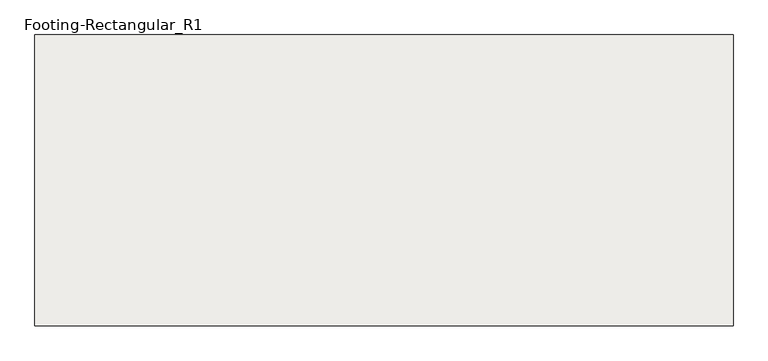
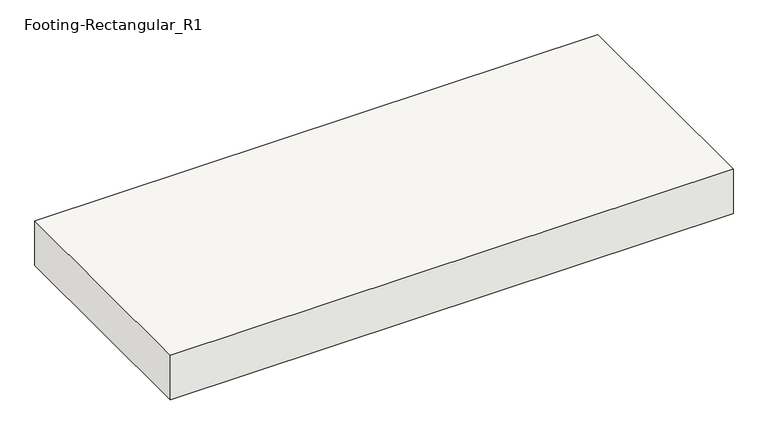
"""IFC4 building model written with IfcOpenShell, lengths in millimetres: slab geometry, Footing-Rectangular_R1 : H_SF_AR_S18_W6000xL2500xT500_Bitumen_F4."""

from ifc_helpers import new_model, si_unit, frame, origin, place, context, project, spatial, polyline, outline, extrude, source, transform, mapped, element, save


def footing_rectangular_r1_297981ed(model_context):
    return source(origin(), model_context, "Body", "SweptSolid", [
        extrude(outline(polyline([(3000.0, 1250.0), (3000.0, -1250.0), (-3000.0, -1250.0), (-3000.0, 1250.0), (3000.0, 1250.0)])), frame((0.0, 0.0, -500.0), z_axis=(0.0, 0.0, 1.0), x_axis=(1.0, 0.0, 0.0)), (0.0, 0.0, 1.0), 500.0),
    ])


if __name__ == "__main__":
    model = new_model("IFC4")
    model_context = context("Model", 3, world=origin())
    ifc_project = project(units=[si_unit("LENGTHUNIT", "METRE", prefix="MILLI")], contexts=[model_context])
    site = spatial("IfcSite", under=ifc_project)
    building = spatial("IfcBuilding", under=site)
    placement = place(None, origin())
    footing_rectangular_r1_shape = footing_rectangular_r1_297981ed(model_context)
    element("IfcSlab", 1, ObjectType="Footing-Rectangular_R1 : H_SF_AR_S18_W6000xL2500xT500_Bitumen_F4", at=placement, inside=building, context=model_context, shape_type="MappedRepresentation", body=[
        mapped(footing_rectangular_r1_shape, transform((0.0, 0.0, 0.0), x_axis=(1.0, 0.0, 0.0), y_axis=(0.0, 1.0, 0.0), z_axis=(0.0, 0.0, 1.0))),
    ])
    save(model, "model.ifc")

# Revit data of these elements
# Type "Footing-Rectangular_R1 : H_SF_AR_S18_W6000xL2500xT500_Bitumen_F4"
#   Type Mark = "F4"
#   Top bar = "D25@300"
#   Description = "UG Shallow Foundation"
#   Bottom bar = "D20@300"
#   Width = 6000 mm
#   Length = 2500 mm
#   Foundation Thickness = 500 mm
#   Structural Material [instance default] = none
#   Assembly Code = ""
